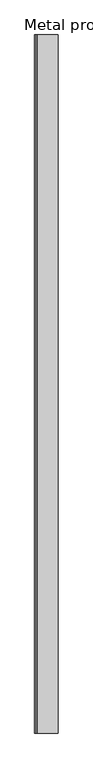
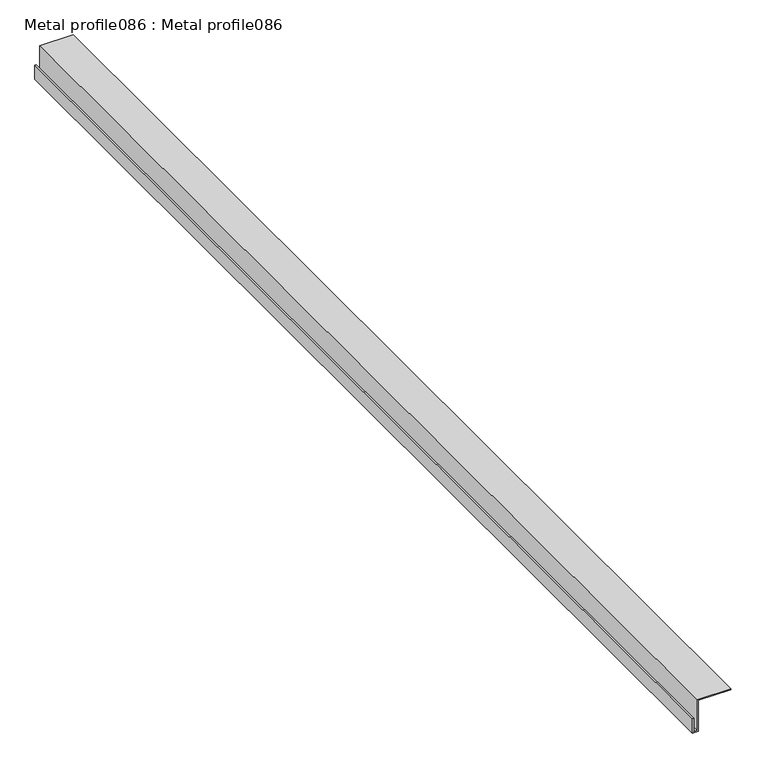
"""IFC4 building model written with IfcOpenShell, lengths in millimetres: proxy geometry, Metal profile086 : Metal profile086."""

import ifcopenshell
import ifcopenshell.guid

model = None  # the IFC model being written
_history = None  # IfcOwnerHistory: only IFC2X3 demands one
_inside = {}  # id of a spatial element -> (the spatial element, [elements in it])
_under = {}  # id of a project, library or spatial element -> (it, [spatial elements below it])
_declared = {}  # id of a project -> (the project, [libraries it declares])
_typed = {}  # id of a type object -> (the type object, [elements of that type])
_made_of = {}  # id of a material, layer set ... -> (it, [elements and type objects made of it])


def new_model(schema):
    """Start an empty IFC model of exactly this schema.

    Asked for "IFC4X3", IfcOpenShell would pick the latest addendum, in which some entities
    have other attributes; the version numbers below select the first issue.
    IFC2X3 requires an IfcOwnerHistory on every rooted entity: one is made here for all.
    """
    global model, _history
    if schema == "IFC4X3":
        model = ifcopenshell.file(schema_version=(4, 3, 0, 0))
    else:
        model = ifcopenshell.file(schema=schema)
    _inside.clear()
    _under.clear()
    _declared.clear()
    _typed.clear()
    _made_of.clear()
    _history = None
    if model.schema == "IFC2X3":
        org = make("IfcOrganization", Name="unknown")
        user = make(
            "IfcPersonAndOrganization",
            ThePerson=make("IfcPerson", FamilyName="unknown"),
            TheOrganization=org,
        )
        app = make(
            "IfcApplication",
            ApplicationDeveloper=org,
            Version="unknown",
            ApplicationFullName="unknown",
            ApplicationIdentifier="unknown",
        )
        _history = make(
            "IfcOwnerHistory",
            OwningUser=user,
            OwningApplication=app,
            ChangeAction="ADDED",
            CreationDate=0,
        )
    return model


def make(cls, **values):
    """One entity of the class cls with the attributes given. An attribute that is None is left unset."""
    return model.create_entity(
        cls, **{name: value for name, value in values.items() if value is not None}
    )


def rooted(cls, **values):
    """An entity with a GlobalId (a new one), such as an element, a storey or a relation."""
    return make(cls, GlobalId=ifcopenshell.guid.new(), OwnerHistory=_history, **values)


def si_unit(unit_type, name, prefix=None):
    """IfcSIUnit, for example si_unit("LENGTHUNIT", "METRE", prefix="MILLI")."""
    return make("IfcSIUnit", UnitType=unit_type, Prefix=prefix, Name=name)


def assignment(units):
    """IfcUnitAssignment: the units of a project."""
    return None if units is None else make("IfcUnitAssignment", Units=units)


def point(xyz):
    """IfcCartesianPoint."""
    return None if xyz is None else make("IfcCartesianPoint", Coordinates=xyz)


def direction(xyz):
    """IfcDirection."""
    return None if xyz is None else make("IfcDirection", DirectionRatios=xyz)


def frame(location, z_axis=None, x_axis=None):
    """IfcAxis2Placement3D, a coordinate frame: its origin and axes. An axis left out is left unset."""
    return make(
        "IfcAxis2Placement3D",
        Location=point(location),
        Axis=direction(z_axis),
        RefDirection=direction(x_axis),
    )


def origin():
    """The frame at (0, 0, 0) with its axes left unset."""
    return frame((0.0, 0.0, 0.0))


def place(relative_to, where):
    """IfcLocalPlacement: puts the frame where relative to a parent placement (None: the world)."""
    return make(
        "IfcLocalPlacement", PlacementRelTo=relative_to, RelativePlacement=where
    )


def context(
    kind, dimensions, precision=None, world=None, true_north=None, identifier=None
):
    """IfcGeometricRepresentationContext, for example the 3D "Model" context."""
    return make(
        "IfcGeometricRepresentationContext",
        ContextIdentifier=identifier,
        ContextType=kind,
        CoordinateSpaceDimension=dimensions,
        Precision=precision,
        WorldCoordinateSystem=world,
        TrueNorth=true_north,
    )


def project(units=None, contexts=None):
    """IfcProject with its units and contexts."""
    return rooted(
        "IfcProject",
        Name="project",
        RepresentationContexts=contexts,
        UnitsInContext=assignment(units),
    )


def spatial(cls, under=None, at=None, **own):
    """A site, building, storey or space (cls), placed at a placement, below another one or the project."""
    s = rooted(cls, ObjectPlacement=at, **own)
    if under is not None:
        _under.setdefault(under.id(), (under, []))[1].append(s)
    return s


def polyline(points):
    """IfcPolyline through the points."""
    return make("IfcPolyline", Points=[point(p) for p in points])


def outline(outer, holes=None, kind="AREA"):
    """IfcArbitraryClosedProfileDef: a profile drawn as a closed curve; with holes, ...WithVoids."""
    if holes is None:
        return make("IfcArbitraryClosedProfileDef", ProfileType=kind, OuterCurve=outer)
    return make(
        "IfcArbitraryProfileDefWithVoids",
        ProfileType=kind,
        OuterCurve=outer,
        InnerCurves=holes,
    )


def extrude(swept, where, along, depth):
    """IfcExtrudedAreaSolid: the profile swept, set in the frame where, extruded along a direction by depth."""
    return make(
        "IfcExtrudedAreaSolid",
        SweptArea=swept,
        Position=where,
        ExtrudedDirection=direction(along),
        Depth=depth,
    )


def shape(context_of_items, identifier, shape_type, items):
    """IfcShapeRepresentation: the items that make up one representation, for example the "Body"."""
    return make(
        "IfcShapeRepresentation",
        ContextOfItems=context_of_items,
        RepresentationIdentifier=identifier,
        RepresentationType=shape_type,
        Items=items,
    )


def source(mapping_origin, context_of_items, identifier, shape_type, items):
    """IfcRepresentationMap: a shape defined once, which mapped items show again and again."""
    return make(
        "IfcRepresentationMap",
        MappingOrigin=mapping_origin,
        MappedRepresentation=shape(context_of_items, identifier, shape_type, items),
    )


def transform(
    local_origin,
    x_axis=None,
    y_axis=None,
    z_axis=None,
    scale=None,
    scale2=None,
    scale3=None,
    uniform=True,
):
    """IfcCartesianTransformationOperator3D, or its non-uniform kind. x_axis, y_axis, z_axis: its Axis1, 2, 3."""
    if uniform:
        return make(
            "IfcCartesianTransformationOperator3D",
            Axis1=direction(x_axis),
            Axis2=direction(y_axis),
            LocalOrigin=point(local_origin),
            Scale=scale,
            Axis3=direction(z_axis),
        )
    return make(
        "IfcCartesianTransformationOperator3DnonUniform",
        Axis1=direction(x_axis),
        Axis2=direction(y_axis),
        LocalOrigin=point(local_origin),
        Scale=scale,
        Axis3=direction(z_axis),
        Scale2=scale2,
        Scale3=scale3,
    )


def mapped(mapping_source, mapping_target):
    """IfcMappedItem: shows the shape of a source again, moved by a transform."""
    return make(
        "IfcMappedItem", MappingSource=mapping_source, MappingTarget=mapping_target
    )


def made_of(thing, what):
    """Note that an element or type object is made of a material, layer set ...; save() writes the relation."""
    if what is not None:
        _made_of.setdefault(what.id(), (what, []))[1].append(thing)
    return thing


def element(
    cls,
    number,
    at=None,
    inside=None,
    cuts=None,
    type_object=None,
    material=None,
    context=None,
    identifier="Body",
    shape_type=None,
    held_by="IfcProductDefinitionShape",
    body=None,
    shapes=None,
    **own,
):
    """One element of the class cls, such as IfcWall. Its Tag is "e" and its number.

    at: its placement. inside: the storey or other place that contains it. cuts: it is an
    opening in that element (IfcRelVoidsElement). A single representation is given by context,
    identifier, shape_type and body (its items); several are given by shapes. held_by: the class
    of the entity that holds the representations. save() writes the other relations.
    """
    e = rooted(cls, Tag="e%d" % number, ObjectPlacement=at, **own)
    if body is not None:
        shapes = [shape(context, identifier, shape_type, body)]
    if shapes is not None:
        e.Representation = make(held_by, Representations=shapes)
    if inside is not None:
        _inside.setdefault(inside.id(), (inside, []))[1].append(e)
    if cuts is not None:
        rooted(
            "IfcRelVoidsElement", RelatingBuildingElement=cuts, RelatedOpeningElement=e
        )
    if type_object is not None:
        _typed.setdefault(type_object.id(), (type_object, []))[1].append(e)
    return made_of(e, material)


def aggregate(whole, parts):
    """IfcRelAggregates: a whole, such as a stair, and the parts it consists of."""
    return rooted("IfcRelAggregates", RelatingObject=whole, RelatedObjects=parts)


def save(model, path):
    """Write the relations noted so far, then the file.

    IfcRelAggregates (storeys below a building ...), IfcRelContainedInSpatialStructure (elements
    in a storey), IfcRelDefinesByType, IfcRelAssociatesMaterial and IfcRelDeclares: one each for
    every whole, place, type object, material and project.
    """
    for whole, parts in _under.values():
        aggregate(whole, parts)
    for where, things in _inside.values():
        rooted(
            "IfcRelContainedInSpatialStructure",
            RelatedElements=things,
            RelatingStructure=where,
        )
    for kind, things in _typed.values():
        rooted("IfcRelDefinesByType", RelatedObjects=things, RelatingType=kind)
    for what, things in _made_of.values():
        rooted("IfcRelAssociatesMaterial", RelatedObjects=things, RelatingMaterial=what)
    for by, libraries in _declared.values():
        rooted("IfcRelDeclares", RelatingContext=by, RelatedDefinitions=libraries)
    model.write(path)


def metal_profile086_metal_profile086_d3e08d76(model_context):
    return source(origin(), model_context, "Body", "SweptSolid", [
        extrude(outline(polyline([(42539.036776, -2413.4999158), (42539.036776, -2403.0365369), (42596.146151, -2403.0365369), (42596.146151, -2346.3602674), (42598.146151, -2346.3602674), (42598.146151, -2405.0365369), (42541.036776, -2405.0365369), (42541.036776, -2411.4999158), (42565.411776, -2411.4999158), (42565.411776, -2413.4999158), (42539.036776, -2413.4999158)])), frame((0.0, -1052.8906574, 0.0), z_axis=(0.0, 1.0, 0.0), x_axis=(0.0, 0.0, 1.0)), (0.0, 0.0, 1.0), 2000.0),
    ])


if __name__ == "__main__":
    model = new_model("IFC4")
    model_context = context("Model", 3, world=origin())
    ifc_project = project(units=[si_unit("LENGTHUNIT", "METRE", prefix="MILLI")], contexts=[model_context])
    site = spatial("IfcSite", under=ifc_project)
    building = spatial("IfcBuilding", under=site)
    placement = place(None, origin())
    metal_profile086_metal_profile086_shape = metal_profile086_metal_profile086_d3e08d76(model_context)
    element("IfcBuildingElementProxy", 1, Name="Metal profile086 : Metal profile086", ObjectType="Metal profile086 : Metal profile086", at=placement, inside=building, context=model_context, shape_type="MappedRepresentation", body=[
        mapped(metal_profile086_metal_profile086_shape, transform((0.0, 0.0, 0.0), x_axis=(1.0, 0.0, 0.0), y_axis=(0.0, 1.0, 0.0), z_axis=(0.0, 0.0, 1.0))),
    ])
    save(model, "model.ifc")

# Revit data of these elements
# Type "Metal profile086 : Metal profile086"
#   NameOverride = "Metal profile086"
# Element 1 (IfcBuildingElementProxy, "Metal profile086 : Metal profile086")
#   Materials on its faces: "ANGLE TRIM"
# Materials
#   "ANGLE TRIM": class "Unassigned", colour RGB 250 255 0, transparency 0
